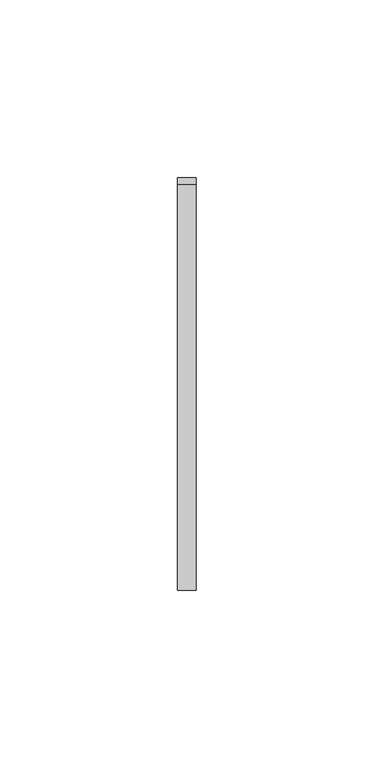
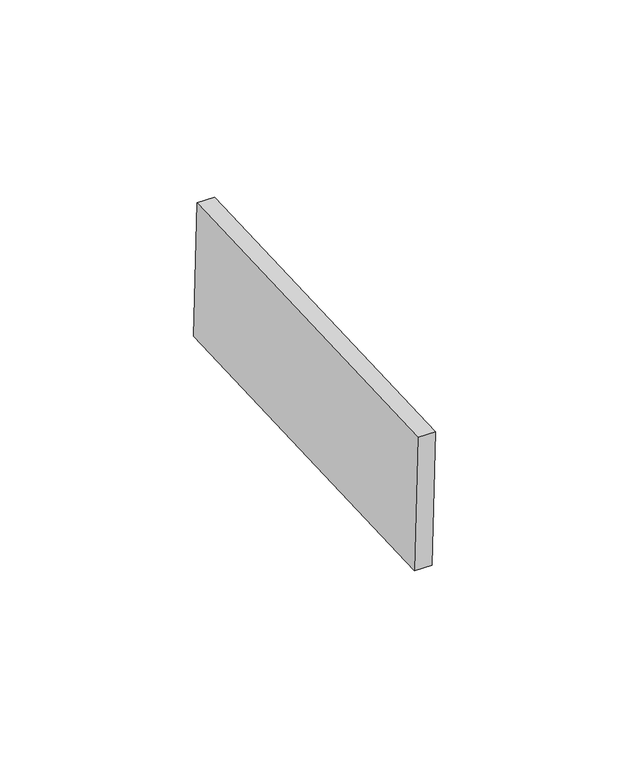
"""IFC4 building model written with IfcOpenShell, lengths in millimetres: proxy geometry, Inner panel:Inner panel:1:Inner panel:1 : Inner panel:Inner panel:300324:2:Inner panel:1:Inner panel:1 : Inner panel:Inner panel:300324:2 : Inner panel:Inner panel:1:Inner panel:1 : Inner panel:Inner panel:300324:300043:89 : Inner panel:Inner panel:1:Inner panel:1 : Inner panel:Inner panel:300324:2:Inner panel:1:Inner panel:1 : Inner panel:Inner panel:300324:2 : Inner panel:Inner panel:1:Inner panel:1 : Inner panel:Inner panel:300324:300043:308120."""

from ifc_helpers import new_model, si_unit, frame, origin, place, context, project, spatial, polyline, outline, extrude, source, transform, mapped, element, save


def generic_models_9ef9dd19(model_context):
    return source(origin(), model_context, "Body", "SweptSolid", [
        extrude(outline(polyline([(0.0, -114.2999999), (0.0, 0.0), (5.2138089, 0.0), (5.2138089, -114.2999999), (0.0, -114.2999999)])), frame((592717.395117, -568168.273882, 8806.9397902), z_axis=(0.0, -0.04163054471215927, 0.9991330730923529), x_axis=(-1.0, 0.0, 0.0)), (0.0, 0.0, 1.0), 43.2233908),
    ])


if __name__ == "__main__":
    model = new_model("IFC4")
    model_context = context("Model", 3, world=origin())
    ifc_project = project(units=[si_unit("LENGTHUNIT", "METRE", prefix="MILLI")], contexts=[model_context])
    site = spatial("IfcSite", under=ifc_project)
    building = spatial("IfcBuilding", under=site)
    placement = place(None, origin())
    generic_models_shape = generic_models_9ef9dd19(model_context)
    element("IfcBuildingElementProxy", 1, Name="Inner panel:Inner panel:1:Inner panel:1 : Inner panel:Inner panel:300324:2:Inner panel:1:Inner panel:1 : Inner panel:Inner panel:300324:2 : Inner panel:Inner panel:1:Inner panel:1 : Inner panel:Inner panel:300324:300043:89 : Inner panel:Inner panel:1:Inner panel:1 : Inner panel:Inner panel:300324:2:Inner panel:1:Inner panel:1 : Inner panel:Inner panel:300324:2 : Inner panel:Inner panel:1:Inner panel:1 : Inner panel:Inner panel:300324:300043:308120", ObjectType="Inner panel:Inner panel:1:Inner panel:1 : Inner panel:Inner panel:300324:2:Inner panel:1:Inner panel:1 : Inner panel:Inner panel:300324:2 : Inner panel:Inner panel:1:Inner panel:1 : Inner panel:Inner panel:300324:300043:89 : Inner panel:Inner panel:1:Inner panel:1 : Inner panel:Inner panel:300324:2:Inner panel:1:Inner panel:1 : Inner panel:Inner panel:300324:2 : Inner panel:Inner panel:1:Inner panel:1 : Inner panel:Inner panel:300324:300043:308120", at=placement, inside=building, context=model_context, shape_type="MappedRepresentation", body=[
        mapped(generic_models_shape, transform((0.0, 0.0, 0.0), x_axis=(1.0, 0.0, 0.0), y_axis=(0.0, 1.0, 0.0), z_axis=(0.0, 0.0, 1.0))),
    ])
    save(model, "model.ifc")

# Revit data of these elements
# Type "Inner panel:Inner panel:1:Inner panel:1 : Inner panel:Inner panel:300324:2:Inner panel:1:Inner panel:1 : Inner panel:Inner panel:300324:2 : Inner panel:Inner panel:1:Inner panel:1 : Inner panel:Inner panel:300324:300043:89 : Inner panel:Inner panel:1:Inner panel:1 : Inner panel:Inner panel:300324:2:Inner panel:1:Inner panel:1 : Inner panel:Inner panel:300324:2 : Inner panel:Inner panel:1:Inner panel:1 : Inner panel:Inner panel:300324:300043:308120"
#   NameOverride = "Inner panel:Inner panel:1:Inner panel:1 : Inner panel:Inner panel:300324:2:Inner panel:1:Inner panel:1 : Inner panel:Inner panel:300324:2 : Inner panel:Inner panel:1:Inner panel:1 : Inner panel:Inner panel:300324:300043:308120"
#   ObjectTypeOverride = "Inner panel:1:Inner panel:1 : Inner panel:Inner panel:300324:2 : Inner panel:Inner panel:1:Inner panel:1 : Inner panel:Inner panel:300324:300043"
#   Reference = "Inner panel"
#   Tag = "308120"
# Element 1 (IfcBuildingElementProxy, "Inner panel:Inner panel:1:Inner panel:1 : Inner panel:Inner panel:300324:2:Inner panel:1:Inner panel:1 : Inner panel:Inner panel:300324:2 : Inner panel:Inner panel:1:Inner panel:1 : Inner panel:Inner panel:300324:300043:89 : Inner panel:Inner panel:1:Inner panel:1 : Inner panel:Inner panel:300324:2:Inner panel:1:Inner panel:1 : Inner panel:Inner panel:300324:2 : Inner panel:Inner panel:1:Inner panel:1 : Inner panel:Inner panel:300324:300043:308120")
#   Materials on its faces: "SLIDING CLIP"
# Materials
#   "SLIDING CLIP": class "Generic", colour RGB 120 120 120, transparency 0, Cost = 0
